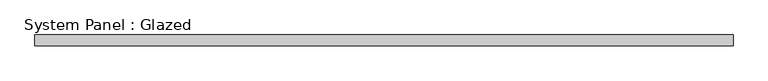
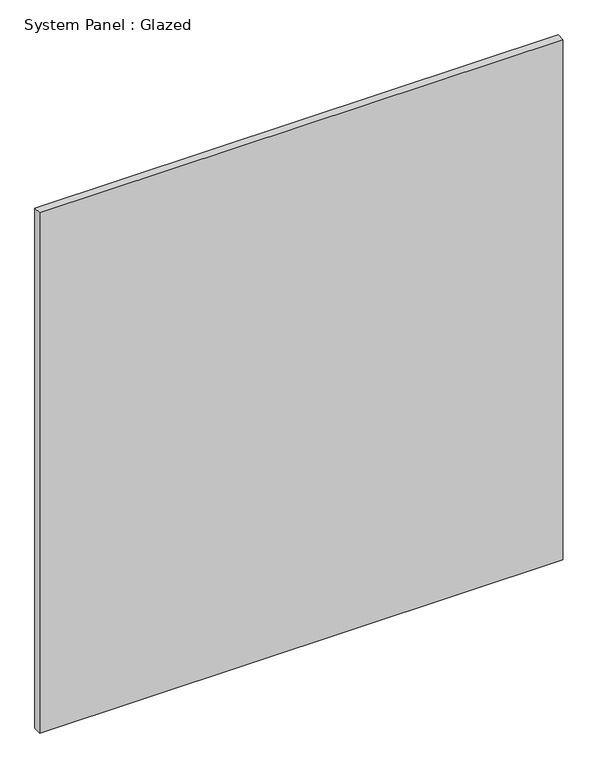
"""IFC4 building model written with IfcOpenShell, lengths in millimetres: plate geometry, System Panel : Glazed."""

from ifc_helpers import new_model, si_unit, origin, origin_with_axes, place, context, project, spatial, polyline, outline, extrude, source, transform, mapped, element, save


def system_panel_glazed_bde8bca4(model_context):
    return source(origin(), model_context, "Body", "SweptSolid", [
        extrude(outline(polyline([(807.8178526, 24.5), (-807.8178526, 24.5), (-807.8178526, 49.5), (807.8178526, 49.5), (807.8178526, 24.5)])), origin_with_axes(), (0.0, 0.0, 1.0), 1698.3122923),
    ])


if __name__ == "__main__":
    model = new_model("IFC4")
    model_context = context("Model", 3, world=origin())
    ifc_project = project(units=[si_unit("LENGTHUNIT", "METRE", prefix="MILLI")], contexts=[model_context])
    site = spatial("IfcSite", under=ifc_project)
    building = spatial("IfcBuilding", under=site)
    placement = place(None, origin())
    system_panel_glazed_shape = system_panel_glazed_bde8bca4(model_context)
    element("IfcPlate", 1, ObjectType="System Panel : Glazed", at=placement, inside=building, context=model_context, shape_type="MappedRepresentation", body=[
        mapped(system_panel_glazed_shape, transform((0.0, 0.0, 0.0), x_axis=(1.0, 0.0, 0.0), y_axis=(0.0, 1.0, 0.0), z_axis=(0.0, 0.0, 1.0))),
    ])
    save(model, "model.ifc")

# Revit data of these elements
# Element 1 (IfcPlate, "System Panel : Glazed")
#   Materials on its faces: "Glass"
# Materials
#   "Glass": class "Glass", colour RGB 218 227 224, transparency 0.85, Description = "Soda Lime Glass", Cost = 0
